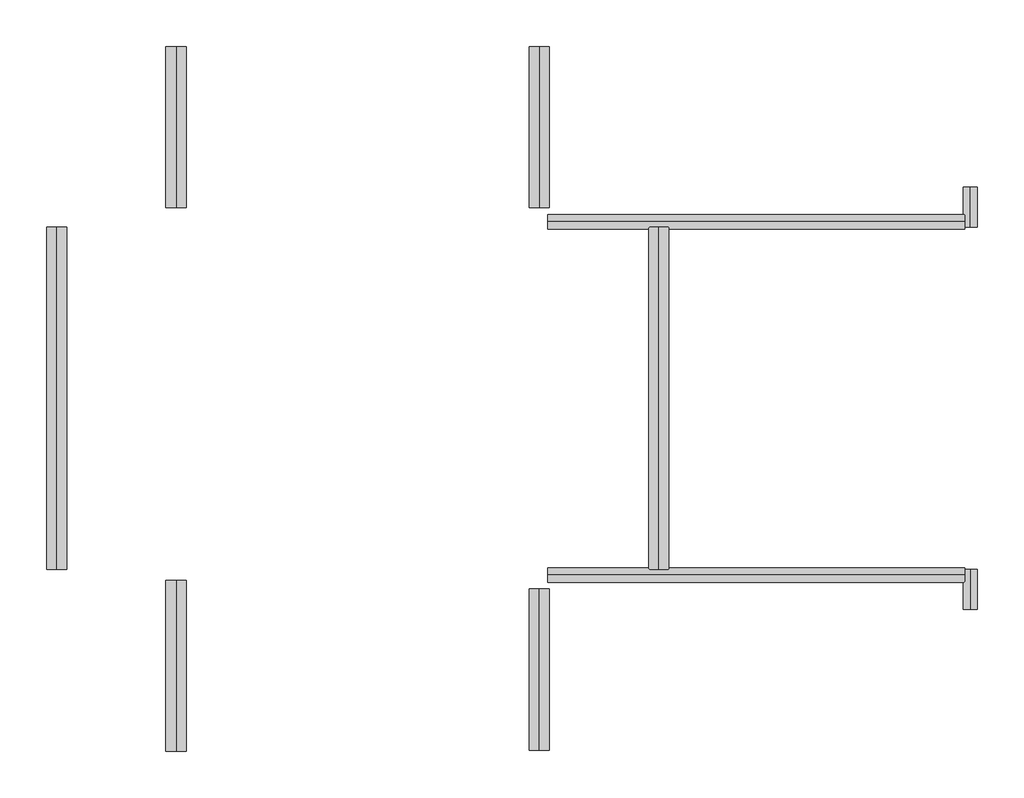
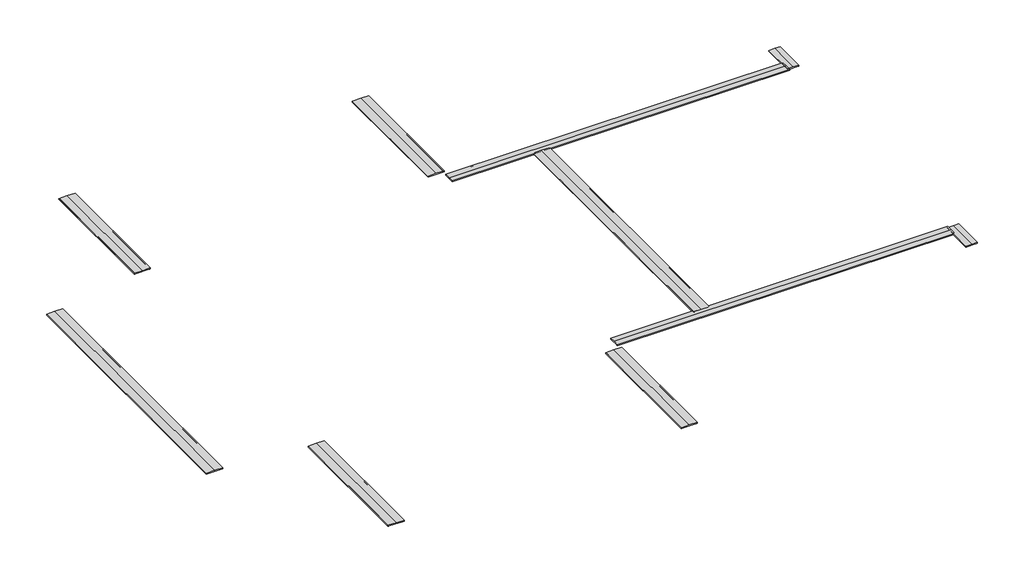
# One storey: 10 proxies.
"""IFC4 building model written with IfcOpenShell, lengths in millimetres."""

from ifc_helpers import new_model, si_unit, frame, origin, place, context, project, spatial, polyline, circle_curve, element, save
from ifc_brep_helpers import plane_surface, revolved_surface, advanced_brep

model = new_model("IFC4")

# Units and contexts
model_context = context("Model", 3, world=origin())
ifc_project = project(units=[si_unit("LENGTHUNIT", "METRE", prefix="MILLI")], contexts=[model_context])

# Site, building, storey
site = spatial("IfcSite", under=ifc_project)
building = spatial("IfcBuilding", under=site)
storey = spatial("IfcBuildingStorey", under=building, Name="AUXILIAR-Peto", Elevation=3030.0)

# Proxies
placement = place(None, origin())
element("IfcBuildingElementProxy", 1, Name="Wall Sweeps", at=placement, inside=storey, context=model_context, shape_type="AdvancedBrep", body=[
    advanced_brep(
    [(-12225.0, -232.5, 3060.0), (-11975.0, -232.5, 3064.3637662), (-11725.0, -232.5, 3060.0), (-11725.0, -232.5, 3030.0), (-11739.8467624, -232.5, 3030.0), (-11754.8467624, -232.5, 3030.0), (-11770.0, -232.5, 3030.0), (-12180.0, -232.5, 3030.0), (-12195.1532376, -232.5, 3030.0), (-12210.1532376, -232.5, 3030.0), (-12225.0, -232.5, 3030.0), (-12225.0, -4252.5, 3060.0), (-12225.0, -4252.5, 3030.0), (-12210.1532376, -4252.5, 3030.0), (-12195.1532376, -4252.5, 3030.0), (-12180.0, -4252.5, 3030.0), (-11770.0, -4252.5, 3030.0), (-11754.8467624, -4252.5, 3030.0), (-11739.8467624, -4252.5, 3030.0), (-11725.0, -4252.5, 3030.0), (-11725.0, -4252.5, 3060.0), (-11975.0, -4252.5, 3064.3637662)],
    [
        (0, 1),
        (1, 2),
        (2, 3),
        (3, 4),
        (4, 5, circle_curve(frame((-11747.3467624, -232.5, 3030.0), z_axis=(0.0, -1.0, 0.0), x_axis=(1.0, 0.0, 0.0)), 7.5)),
        (5, 6),
        (6, 7),
        (7, 8),
        (8, 9, circle_curve(frame((-12202.6532376, -232.5, 3030.0), z_axis=(0.0, -1.0, 0.0), x_axis=(1.0, 0.0, 0.0)), 7.5)),
        (9, 10),
        (10, 0),
        (11, 12),
        (12, 13),
        (13, 14, circle_curve(frame((-12202.6532376, -4252.5, 3030.0), z_axis=(0.0, 1.0, 0.0), x_axis=(1.0, 0.0, 0.0)), 7.5)),
        (14, 15),
        (15, 16),
        (16, 17),
        (17, 18, circle_curve(frame((-11747.3467624, -4252.5, 3030.0), z_axis=(0.0, 1.0, 0.0), x_axis=(1.0, 0.0, 0.0)), 7.5)),
        (18, 19),
        (19, 20),
        (20, 21),
        (21, 11),
        (0, 11),
        (21, 1),
        (20, 2),
        (19, 3),
        (18, 4),
        (17, 5),
        (14, 8),
        (13, 9),
        (12, 10),
    ],
    [
        plane_surface(frame((-12225.9879384, -232.5, 3030.0), z_axis=(0.0, 1.0, 0.0), x_axis=(0.0, 0.0, -1.0))),
        plane_surface(frame((-12225.9879384, -4252.5, 3030.0), z_axis=(0.0, -1.0, 0.0), x_axis=(0.0, 0.0, -1.0))),
        plane_surface(frame((-12225.0, -232.5, 3060.0), z_axis=(-0.01745240643728998, 0.0, 0.9998476951563912), x_axis=(0.0, -1.0, 0.0))),
        plane_surface(frame((-11975.0, -232.5, 3064.3637662), z_axis=(0.017452406437287852, 0.0, 0.9998476951563912), x_axis=(0.0, -1.0, 0.0))),
        plane_surface(frame((-11725.0, -232.5, 3060.0), z_axis=(1.0, 0.0, 0.0), x_axis=(0.0, -1.0, 0.0))),
        plane_surface(frame((-11725.0, -232.5, 3030.0), z_axis=(0.0, 0.0, -1.0), x_axis=(0.0, -1.0, 0.0))),
        revolved_surface(polyline([(-11739.8467624, -4252.5, 3030.0), (-11739.8467624, -232.5, 3030.0)]), (-11747.3467624, -232.5, 3030.0), (0.0, -1.0, 0.0)),
        plane_surface(frame((-11754.8467624, -232.5, 3030.0), z_axis=(0.0, 0.0, -1.0), x_axis=(0.0, -1.0, 0.0))),
        revolved_surface(polyline([(-12195.1532376, -4252.5, 3030.0), (-12195.1532376, -232.5, 3030.0)]), (-12202.6532376, -232.5, 3030.0), (0.0, -1.0, 0.0)),
        plane_surface(frame((-12210.1532376, -232.5, 3030.0), z_axis=(0.0, 0.0, -1.0), x_axis=(0.0, -1.0, 0.0))),
        plane_surface(frame((-12225.0, -232.5, 3030.0), z_axis=(-1.0, 0.0, 0.0), x_axis=(0.0, -1.0, 0.0))),
    ],
    [
        (0, [[1, 2, 3, 4, 5, 6, 7, 8, 9, 10, 11]]),
        (1, [[12, 13, 14, 15, 16, 17, 18, 19, 20, 21, 22]]),
        (2, [[-1, 23, -22, 24]]),
        (3, [[-2, -24, -21, 25]]),
        (4, [[-3, -25, -20, 26]]),
        (5, [[-4, -26, -19, 27]]),
        (6, [[-5, -27, -18, 28]]),
        (7, [[-8, -7, -6, -28, -17, -16, -15, 29]]),
        (8, [[-9, -29, -14, 30]]),
        (9, [[-10, -30, -13, 31]]),
        (10, [[-11, -31, -12, -23]]),
    ],
),
])
element("IfcBuildingElementProxy", 2, Name="Wall Sweeps", at=placement, inside=storey, context=model_context, shape_type="AdvancedBrep", body=[
    advanced_brep(
    [(-20775.0, -232.5, 3060.0), (-20775.0, -232.5, 3030.0), (-20789.8467624, -232.5, 3030.0), (-20804.8467624, -232.5, 3030.0), (-20820.0, -232.5, 3030.0), (-21230.0, -232.5, 3030.0), (-21245.1532376, -232.5, 3030.0), (-21260.1532376, -232.5, 3030.0), (-21275.0, -232.5, 3030.0), (-21275.0, -232.5, 3060.0), (-21025.0, -232.5, 3064.3637662), (-20775.0, -4252.5, 3060.0), (-21025.0, -4252.5, 3064.3637662), (-21275.0, -4252.5, 3060.0), (-21275.0, -4252.5, 3030.0), (-21260.1532376, -4252.5, 3030.0), (-21245.1532376, -4252.5, 3030.0), (-21230.0, -4252.5, 3030.0), (-20820.0, -4252.5, 3030.0), (-20804.8467624, -4252.5, 3030.0), (-20789.8467624, -4252.5, 3030.0), (-20775.0, -4252.5, 3030.0)],
    [
        (0, 1),
        (1, 2),
        (2, 3, circle_curve(frame((-20797.3467624, -232.5, 3030.0), z_axis=(0.0, -1.0, 0.0), x_axis=(-1.0, 0.0, 0.0)), 7.5)),
        (3, 4),
        (4, 5),
        (5, 6),
        (6, 7, circle_curve(frame((-21252.6532376, -232.5, 3030.0), z_axis=(0.0, -1.0, 0.0), x_axis=(-1.0, 0.0, 0.0)), 7.5)),
        (7, 8),
        (8, 9),
        (9, 10),
        (10, 0),
        (11, 12),
        (12, 13),
        (13, 14),
        (14, 15),
        (15, 16, circle_curve(frame((-21252.6532376, -4252.5, 3030.0), z_axis=(0.0, 1.0, 0.0), x_axis=(-1.0, 0.0, 0.0)), 7.5)),
        (16, 17),
        (17, 18),
        (18, 19),
        (19, 20, circle_curve(frame((-20797.3467624, -4252.5, 3030.0), z_axis=(0.0, 1.0, 0.0), x_axis=(-1.0, 0.0, 0.0)), 7.5)),
        (20, 21),
        (21, 11),
        (0, 11),
        (21, 1),
        (20, 2),
        (19, 3),
        (16, 6),
        (15, 7),
        (14, 8),
        (13, 9),
        (12, 10),
    ],
    [
        plane_surface(frame((-21685.9879384, -232.5, 3030.0), z_axis=(0.0, 1.0, 0.0), x_axis=(0.0, 0.0, -1.0))),
        plane_surface(frame((-21685.9879384, -4252.5, 3030.0), z_axis=(0.0, -1.0, 0.0), x_axis=(0.0, 0.0, -1.0))),
        plane_surface(frame((-20775.0, -232.5, 3060.0), z_axis=(1.0, 0.0, 0.0), x_axis=(0.0, -1.0, 0.0))),
        plane_surface(frame((-20775.0, -232.5, 3030.0), z_axis=(0.0, 0.0, -1.0), x_axis=(0.0, -1.0, 0.0))),
        revolved_surface(polyline([(-20804.8467624, -4252.5, 3030.0), (-20804.8467624, -232.5, 3030.0)]), (-20797.3467624, -232.5, 3030.0), (0.0, -1.0, 0.0)),
        plane_surface(frame((-20804.8467624, -232.5, 3030.0), z_axis=(0.0, 0.0, -1.0), x_axis=(0.0, -1.0, 0.0))),
        revolved_surface(polyline([(-21260.1532376, -4252.5, 3030.0), (-21260.1532376, -232.5, 3030.0)]), (-21252.6532376, -232.5, 3030.0), (0.0, -1.0, 0.0)),
        plane_surface(frame((-21260.1532376, -232.5, 3030.0), z_axis=(0.0, 0.0, -1.0), x_axis=(0.0, -1.0, 0.0))),
        plane_surface(frame((-21275.0, -232.5, 3030.0), z_axis=(-1.0, 0.0, 0.0), x_axis=(0.0, -1.0, 0.0))),
        plane_surface(frame((-21275.0, -232.5, 3060.0), z_axis=(-0.017452406437287852, 0.0, 0.9998476951563912), x_axis=(0.0, -1.0, 0.0))),
        plane_surface(frame((-21025.0, -232.5, 3064.3637662), z_axis=(0.01745240643728998, 0.0, 0.9998476951563912), x_axis=(0.0, -1.0, 0.0))),
    ],
    [
        (0, [[1, 2, 3, 4, 5, 6, 7, 8, 9, 10, 11]]),
        (1, [[12, 13, 14, 15, 16, 17, 18, 19, 20, 21, 22]]),
        (2, [[-1, 23, -22, 24]]),
        (3, [[-2, -24, -21, 25]]),
        (4, [[-3, -25, -20, 26]]),
        (5, [[-6, -5, -4, -26, -19, -18, -17, 27]]),
        (6, [[-7, -27, -16, 28]]),
        (7, [[-8, -28, -15, 29]]),
        (8, [[-9, -29, -14, 30]]),
        (9, [[-10, -30, -13, 31]]),
        (10, [[-11, -31, -12, -23]]),
    ],
),
])
element("IfcBuildingElementProxy", 3, Name="Wall Sweeps", at=placement, inside=storey, context=model_context, shape_type="AdvancedBrep", body=[
    advanced_brep(
    [(-12225.0, -17767.5, 3060.0), (-12225.0, -17767.5, 3030.0), (-12210.1532376, -17767.5, 3030.0), (-12195.1532376, -17767.5, 3030.0), (-12180.0, -17767.5, 3030.0), (-11770.0, -17767.5, 3030.0), (-11754.8467624, -17767.5, 3030.0), (-11739.8467624, -17767.5, 3030.0), (-11725.0, -17767.5, 3030.0), (-11725.0, -17767.5, 3060.0), (-11975.0, -17767.5, 3064.3637662), (-12225.0, -13747.5, 3060.0), (-11975.0, -13747.5, 3064.3637662), (-11725.0, -13747.5, 3060.0), (-11725.0, -13747.5, 3030.0), (-11739.8467624, -13747.5, 3030.0), (-11754.8467624, -13747.5, 3030.0), (-11770.0, -13747.5, 3030.0), (-12180.0, -13747.5, 3030.0), (-12195.1532376, -13747.5, 3030.0), (-12210.1532376, -13747.5, 3030.0), (-12225.0, -13747.5, 3030.0)],
    [
        (0, 1),
        (1, 2),
        (2, 3, circle_curve(frame((-12202.6532376, -17767.5, 3030.0), z_axis=(0.0, 1.0, 0.0), x_axis=(1.0, 0.0, 0.0)), 7.5)),
        (3, 4),
        (4, 5),
        (5, 6),
        (6, 7, circle_curve(frame((-11747.3467624, -17767.5, 3030.0), z_axis=(0.0, 1.0, 0.0), x_axis=(1.0, 0.0, 0.0)), 7.5)),
        (7, 8),
        (8, 9),
        (9, 10),
        (10, 0),
        (11, 12),
        (12, 13),
        (13, 14),
        (14, 15),
        (15, 16, circle_curve(frame((-11747.3467624, -13747.5, 3030.0), z_axis=(0.0, -1.0, 0.0), x_axis=(1.0, 0.0, 0.0)), 7.5)),
        (16, 17),
        (17, 18),
        (18, 19),
        (19, 20, circle_curve(frame((-12202.6532376, -13747.5, 3030.0), z_axis=(0.0, -1.0, 0.0), x_axis=(1.0, 0.0, 0.0)), 7.5)),
        (20, 21),
        (21, 11),
        (0, 11),
        (21, 1),
        (20, 2),
        (19, 3),
        (16, 6),
        (15, 7),
        (14, 8),
        (13, 9),
        (12, 10),
    ],
    [
        plane_surface(frame((-12225.9879384, -17767.5, 3030.0), z_axis=(0.0, -1.0, 0.0), x_axis=(0.0, 0.0, 1.0))),
        plane_surface(frame((-12225.9879384, -13747.5, 3030.0), z_axis=(0.0, 1.0, 0.0), x_axis=(0.0, 0.0, 1.0))),
        plane_surface(frame((-12225.0, -17767.5, 3060.0), z_axis=(-1.0, 0.0, 0.0), x_axis=(0.0, 1.0, 0.0))),
        plane_surface(frame((-12225.0, -17767.5, 3030.0), z_axis=(0.0, 0.0, -1.0), x_axis=(0.0, 1.0, 0.0))),
        revolved_surface(polyline([(-12195.1532376, -13747.5, 3030.0), (-12195.1532376, -17767.5, 3030.0)]), (-12202.6532376, -17767.5, 3030.0), (0.0, 1.0, 0.0)),
        plane_surface(frame((-12195.1532376, -17767.5, 3030.0), z_axis=(0.0, 0.0, -1.0), x_axis=(0.0, 1.0, 0.0))),
        revolved_surface(polyline([(-11739.8467624, -13747.5, 3030.0), (-11739.8467624, -17767.5, 3030.0)]), (-11747.3467624, -17767.5, 3030.0), (0.0, 1.0, 0.0)),
        plane_surface(frame((-11739.8467624, -17767.5, 3030.0), z_axis=(0.0, 0.0, -1.0), x_axis=(0.0, 1.0, 0.0))),
        plane_surface(frame((-11725.0, -17767.5, 3030.0), z_axis=(1.0, 0.0, 0.0), x_axis=(0.0, 1.0, 0.0))),
        plane_surface(frame((-11725.0, -17767.5, 3060.0), z_axis=(0.017452406437287852, 0.0, 0.9998476951563912), x_axis=(0.0, 1.0, 0.0))),
        plane_surface(frame((-11975.0, -17767.5, 3064.3637662), z_axis=(-0.01745240643728998, 0.0, 0.9998476951563912), x_axis=(0.0, 1.0, 0.0))),
    ],
    [
        (0, [[1, 2, 3, 4, 5, 6, 7, 8, 9, 10, 11]]),
        (1, [[12, 13, 14, 15, 16, 17, 18, 19, 20, 21, 22]]),
        (2, [[-1, 23, -22, 24]]),
        (3, [[-2, -24, -21, 25]]),
        (4, [[-3, -25, -20, 26]]),
        (5, [[-6, -5, -4, -26, -19, -18, -17, 27]]),
        (6, [[-7, -27, -16, 28]]),
        (7, [[-8, -28, -15, 29]]),
        (8, [[-9, -29, -14, 30]]),
        (9, [[-10, -30, -13, 31]]),
        (10, [[-11, -31, -12, -23]]),
    ],
),
])
element("IfcBuildingElementProxy", 4, Name="Wall Sweeps", at=placement, inside=storey, context=model_context, shape_type="AdvancedBrep", body=[
    advanced_brep(
    [(-23750.0, -13267.5, 3060.0), (-24000.0, -13267.5, 3064.3637662), (-24250.0, -13267.5, 3060.0), (-24250.0, -13267.5, 3030.0), (-24235.1532376, -13267.5, 3030.0), (-24220.1532376, -13267.5, 3030.0), (-24205.0, -13267.5, 3030.0), (-23795.0, -13267.5, 3030.0), (-23779.8467624, -13267.5, 3030.0), (-23764.8467624, -13267.5, 3030.0), (-23750.0, -13267.5, 3030.0), (-23750.0, -4732.5, 3060.0), (-23750.0, -4732.5, 3030.0), (-23764.8467624, -4732.5, 3030.0), (-23779.8467624, -4732.5, 3030.0), (-23795.0, -4732.5, 3030.0), (-24205.0, -4732.5, 3030.0), (-24220.1532376, -4732.5, 3030.0), (-24235.1532376, -4732.5, 3030.0), (-24250.0, -4732.5, 3030.0), (-24250.0, -4732.5, 3060.0), (-24000.0, -4732.5, 3064.3637662)],
    [
        (0, 1),
        (1, 2),
        (2, 3),
        (3, 4),
        (4, 5, circle_curve(frame((-24227.6532376, -13267.5, 3030.0), z_axis=(0.0, 1.0, 0.0), x_axis=(-1.0, 0.0, 0.0)), 7.5)),
        (5, 6),
        (6, 7),
        (7, 8),
        (8, 9, circle_curve(frame((-23772.3467624, -13267.5, 3030.0), z_axis=(0.0, 1.0, 0.0), x_axis=(-1.0, 0.0, 0.0)), 7.5)),
        (9, 10),
        (10, 0),
        (11, 12),
        (12, 13),
        (13, 14, circle_curve(frame((-23772.3467624, -4732.5, 3030.0), z_axis=(0.0, -1.0, 0.0), x_axis=(-1.0, 0.0, 0.0)), 7.5)),
        (14, 15),
        (15, 16),
        (16, 17),
        (17, 18, circle_curve(frame((-24227.6532376, -4732.5, 3030.0), z_axis=(0.0, -1.0, 0.0), x_axis=(-1.0, 0.0, 0.0)), 7.5)),
        (18, 19),
        (19, 20),
        (20, 21),
        (21, 11),
        (0, 11),
        (21, 1),
        (20, 2),
        (19, 3),
        (18, 4),
        (17, 5),
        (14, 8),
        (13, 9),
        (12, 10),
    ],
    [
        plane_surface(frame((-24660.9879384, -13267.5, 3030.0), z_axis=(0.0, -1.0, 0.0), x_axis=(0.0, 0.0, 1.0))),
        plane_surface(frame((-24660.9879384, -4732.5, 3030.0), z_axis=(0.0, 1.0, 0.0), x_axis=(0.0, 0.0, 1.0))),
        plane_surface(frame((-23750.0, -13267.5, 3060.0), z_axis=(0.01745240643728998, 0.0, 0.9998476951563912), x_axis=(0.0, 1.0, 0.0))),
        plane_surface(frame((-24000.0, -13267.5, 3064.3637662), z_axis=(-0.017452406437287852, 0.0, 0.9998476951563912), x_axis=(0.0, 1.0, 0.0))),
        plane_surface(frame((-24250.0, -13267.5, 3060.0), z_axis=(-1.0, 0.0, 0.0), x_axis=(0.0, 1.0, 0.0))),
        plane_surface(frame((-24250.0, -13267.5, 3030.0), z_axis=(0.0, 0.0, -1.0), x_axis=(0.0, 1.0, 0.0))),
        revolved_surface(polyline([(-24235.1532376, -4732.5, 3030.0), (-24235.1532376, -13267.5, 3030.0)]), (-24227.6532376, -13267.5, 3030.0), (0.0, 1.0, 0.0)),
        plane_surface(frame((-24220.1532376, -13267.5, 3030.0), z_axis=(0.0, 0.0, -1.0), x_axis=(0.0, 1.0, 0.0))),
        revolved_surface(polyline([(-23779.8467624, -4732.5, 3030.0), (-23779.8467624, -13267.5, 3030.0)]), (-23772.3467624, -13267.5, 3030.0), (0.0, 1.0, 0.0)),
        plane_surface(frame((-23764.8467624, -13267.5, 3030.0), z_axis=(0.0, 0.0, -1.0), x_axis=(0.0, 1.0, 0.0))),
        plane_surface(frame((-23750.0, -13267.5, 3030.0), z_axis=(1.0, 0.0, 0.0), x_axis=(0.0, 1.0, 0.0))),
    ],
    [
        (0, [[1, 2, 3, 4, 5, 6, 7, 8, 9, 10, 11]]),
        (1, [[12, 13, 14, 15, 16, 17, 18, 19, 20, 21, 22]]),
        (2, [[-1, 23, -22, 24]]),
        (3, [[-2, -24, -21, 25]]),
        (4, [[-3, -25, -20, 26]]),
        (5, [[-4, -26, -19, 27]]),
        (6, [[-5, -27, -18, 28]]),
        (7, [[-8, -7, -6, -28, -17, -16, -15, 29]]),
        (8, [[-9, -29, -14, 30]]),
        (9, [[-10, -30, -13, 31]]),
        (10, [[-11, -31, -12, -23]]),
    ],
),
])
element("IfcBuildingElementProxy", 5, Name="Wall Sweeps", at=placement, inside=storey, context=model_context, shape_type="AdvancedBrep", body=[
    advanced_brep(
    [(-9250.0, -13267.5, 3060.0), (-9250.0, -13267.5, 3030.0), (-9235.1532376, -13267.5, 3030.0), (-9220.1532376, -13267.5, 3030.0), (-9205.0, -13267.5, 3030.0), (-8795.0, -13267.5, 3030.0), (-8779.8467624, -13267.5, 3030.0), (-8764.8467624, -13267.5, 3030.0), (-8750.0, -13267.5, 3030.0), (-8750.0, -13267.5, 3060.0), (-9000.0, -13267.5, 3064.3637662), (-9250.0, -4732.5, 3060.0), (-9000.0, -4732.5, 3064.3637662), (-8750.0, -4732.5, 3060.0), (-8750.0, -4732.5, 3030.0), (-8764.8467624, -4732.5, 3030.0), (-8779.8467624, -4732.5, 3030.0), (-8795.0, -4732.5, 3030.0), (-9205.0, -4732.5, 3030.0), (-9220.1532376, -4732.5, 3030.0), (-9235.1532376, -4732.5, 3030.0), (-9250.0, -4732.5, 3030.0)],
    [
        (0, 1),
        (1, 2),
        (2, 3, circle_curve(frame((-9227.6532376, -13267.5, 3030.0), z_axis=(0.0, 1.0, 0.0), x_axis=(1.0, 0.0, 0.0)), 7.5)),
        (3, 4),
        (4, 5),
        (5, 6),
        (6, 7, circle_curve(frame((-8772.3467624, -13267.5, 3030.0), z_axis=(0.0, 1.0, 0.0), x_axis=(1.0, 0.0, 0.0)), 7.5)),
        (7, 8),
        (8, 9),
        (9, 10),
        (10, 0),
        (11, 12),
        (12, 13),
        (13, 14),
        (14, 15),
        (15, 16, circle_curve(frame((-8772.3467624, -4732.5, 3030.0), z_axis=(0.0, -1.0, 0.0), x_axis=(1.0, 0.0, 0.0)), 7.5)),
        (16, 17),
        (17, 18),
        (18, 19),
        (19, 20, circle_curve(frame((-9227.6532376, -4732.5, 3030.0), z_axis=(0.0, -1.0, 0.0), x_axis=(1.0, 0.0, 0.0)), 7.5)),
        (20, 21),
        (21, 11),
        (0, 11),
        (21, 1),
        (20, 2),
        (19, 3),
        (16, 6),
        (15, 7),
        (14, 8),
        (13, 9),
        (12, 10),
    ],
    [
        plane_surface(frame((-9250.9879384, -13267.5, 3030.0), z_axis=(0.0, -1.0, 0.0), x_axis=(0.0, 0.0, 1.0))),
        plane_surface(frame((-9250.9879384, -4732.5, 3030.0), z_axis=(0.0, 1.0, 0.0), x_axis=(0.0, 0.0, 1.0))),
        plane_surface(frame((-9250.0, -13267.5, 3060.0), z_axis=(-1.0, 0.0, 0.0), x_axis=(0.0, 1.0, 0.0))),
        plane_surface(frame((-9250.0, -13267.5, 3030.0), z_axis=(0.0, 0.0, -1.0), x_axis=(0.0, 1.0, 0.0))),
        revolved_surface(polyline([(-9220.1532376, -4732.5, 3030.0), (-9220.1532376, -13267.5, 3030.0)]), (-9227.6532376, -13267.5, 3030.0), (0.0, 1.0, 0.0)),
        plane_surface(frame((-9220.1532376, -13267.5, 3030.0), z_axis=(0.0, 0.0, -1.0), x_axis=(0.0, 1.0, 0.0))),
        revolved_surface(polyline([(-8764.8467624, -4732.5, 3030.0), (-8764.8467624, -13267.5, 3030.0)]), (-8772.3467624, -13267.5, 3030.0), (0.0, 1.0, 0.0)),
        plane_surface(frame((-8764.8467624, -13267.5, 3030.0), z_axis=(0.0, 0.0, -1.0), x_axis=(0.0, 1.0, 0.0))),
        plane_surface(frame((-8750.0, -13267.5, 3030.0), z_axis=(1.0, 0.0, 0.0), x_axis=(0.0, 1.0, 0.0))),
        plane_surface(frame((-8750.0, -13267.5, 3060.0), z_axis=(0.017452406437287852, 0.0, 0.9998476951563912), x_axis=(0.0, 1.0, 0.0))),
        plane_surface(frame((-9000.0, -13267.5, 3064.3637662), z_axis=(-0.01745240643728998, 0.0, 0.9998476951563912), x_axis=(0.0, 1.0, 0.0))),
    ],
    [
        (0, [[1, 2, 3, 4, 5, 6, 7, 8, 9, 10, 11]]),
        (1, [[12, 13, 14, 15, 16, 17, 18, 19, 20, 21, 22]]),
        (2, [[-1, 23, -22, 24]]),
        (3, [[-2, -24, -21, 25]]),
        (4, [[-3, -25, -20, 26]]),
        (5, [[-6, -5, -4, -26, -19, -18, -17, 27]]),
        (6, [[-7, -27, -16, 28]]),
        (7, [[-8, -28, -15, 29]]),
        (8, [[-9, -29, -14, 30]]),
        (9, [[-10, -30, -13, 31]]),
        (10, [[-11, -31, -12, -23]]),
    ],
),
])
element("IfcBuildingElementProxy", 6, Name="Wall Sweeps", at=placement, inside=storey, context=model_context, shape_type="AdvancedBrep", body=[
    advanced_brep(
    [(-11770.0, -13222.5, 3060.0), (-11770.0, -13222.5, 3030.0), (-11770.0, -13237.3467624, 3030.0), (-11770.0, -13252.3467624, 3030.0), (-11770.0, -13267.5, 3030.0), (-11770.0, -13537.5, 3030.0), (-11770.0, -13552.6532376, 3030.0), (-11770.0, -13567.6532376, 3030.0), (-11770.0, -13582.5, 3030.0), (-11770.0, -13582.5, 3060.0), (-11770.0, -13402.5, 3063.1419117), (-1380.0, -13222.5, 3060.0), (-1380.0, -13402.5, 3063.1419117), (-1380.0, -13582.5, 3060.0), (-1380.0, -13582.5, 3030.0), (-1380.0, -13567.6532376, 3030.0), (-1380.0, -13552.6532376, 3030.0), (-1380.0, -13252.3467624, 3030.0), (-1380.0, -13237.3467624, 3030.0), (-1380.0, -13222.5, 3030.0)],
    [
        (0, 1),
        (1, 2),
        (2, 3, circle_curve(frame((-11770.0, -13244.8467624, 3030.0), z_axis=(1.0, 0.0, 0.0), x_axis=(0.0, -1.0, 0.0)), 7.5)),
        (3, 4),
        (4, 5),
        (5, 6),
        (6, 7, circle_curve(frame((-11770.0, -13560.1532376, 3030.0), z_axis=(1.0, 0.0, 0.0), x_axis=(0.0, -1.0, 0.0)), 7.5)),
        (7, 8),
        (8, 9),
        (9, 10),
        (10, 0),
        (11, 12),
        (12, 13),
        (13, 14),
        (14, 15),
        (15, 16, circle_curve(frame((-1380.0, -13560.1532376, 3030.0), z_axis=(-1.0, 0.0, 0.0), x_axis=(0.0, -1.0, 0.0)), 7.5)),
        (16, 17),
        (17, 18, circle_curve(frame((-1380.0, -13244.8467624, 3030.0), z_axis=(-1.0, 0.0, 0.0), x_axis=(0.0, -1.0, 0.0)), 7.5)),
        (18, 19),
        (19, 11),
        (0, 11),
        (19, 1),
        (18, 2),
        (17, 3),
        (16, 6),
        (15, 7),
        (14, 8),
        (13, 9),
        (12, 10),
    ],
    [
        plane_surface(frame((-11770.0, -13537.5, 2713.5746534), z_axis=(-1.0, 0.0, 0.0), x_axis=(0.0, 1.0, 0.0))),
        plane_surface(frame((-1380.0, -13537.5, 2713.5746534), z_axis=(1.0, 0.0, 0.0), x_axis=(0.0, 1.0, 0.0))),
        plane_surface(frame((-11770.0, -13222.5, 3060.0), z_axis=(0.0, 1.0, 0.0), x_axis=(1.0, 0.0, 0.0))),
        plane_surface(frame((-11770.0, -13222.5, 3030.0), z_axis=(0.0, 0.0, -1.0), x_axis=(1.0, 0.0, 0.0))),
        revolved_surface(polyline([(-1380.0, -13252.3467624, 3030.0), (-11770.0, -13252.3467624, 3030.0)]), (-11770.0, -13244.8467624, 3030.0), (1.0, 0.0, 0.0)),
        plane_surface(frame((-11770.0, -13252.3467624, 3030.0), z_axis=(0.0, 0.0, -1.0), x_axis=(1.0, 0.0, 0.0))),
        revolved_surface(polyline([(-1380.0, -13567.6532376, 3030.0), (-11770.0, -13567.6532376, 3030.0)]), (-11770.0, -13560.1532376, 3030.0), (1.0, 0.0, 0.0)),
        plane_surface(frame((-11770.0, -13567.6532376, 3030.0), z_axis=(0.0, 0.0, -1.0), x_axis=(1.0, 0.0, 0.0))),
        plane_surface(frame((-11770.0, -13582.5, 3030.0), z_axis=(0.0, -1.0, 0.0), x_axis=(1.0, 0.0, 0.0))),
        plane_surface(frame((-11770.0, -13582.5, 3060.0), z_axis=(0.0, -0.01745240643728671, 0.9998476951563913), x_axis=(1.0, 0.0, 0.0))),
        plane_surface(frame((-11770.0, -13402.5, 3063.1419117), z_axis=(0.0, 0.01745240643728026, 0.9998476951563914), x_axis=(1.0, 0.0, 0.0))),
    ],
    [
        (0, [[1, 2, 3, 4, 5, 6, 7, 8, 9, 10, 11]]),
        (1, [[12, 13, 14, 15, 16, 17, 18, 19, 20]]),
        (2, [[-1, 21, -20, 22]]),
        (3, [[-2, -22, -19, 23]]),
        (4, [[-3, -23, -18, 24]]),
        (5, [[-6, -5, -4, -24, -17, 25]]),
        (6, [[-7, -25, -16, 26]]),
        (7, [[-8, -26, -15, 27]]),
        (8, [[-9, -27, -14, 28]]),
        (9, [[-10, -28, -13, 29]]),
        (10, [[-11, -29, -12, -21]]),
    ],
),
])
element("IfcBuildingElementProxy", 7, Name="Wall Sweeps", at=placement, inside=storey, context=model_context, shape_type="AdvancedBrep", body=[
    advanced_brep(
    [(-1425.0, -13267.5, 3060.0), (-1245.0, -13267.5, 3063.1419117), (-1065.0, -13267.5, 3060.0), (-1065.0, -13267.5, 3030.0), (-1079.8467624, -13267.5, 3030.0), (-1094.8467624, -13267.5, 3030.0), (-1395.1532376, -13267.5, 3030.0), (-1410.1532376, -13267.5, 3030.0), (-1425.0, -13267.5, 3030.0), (-1425.0, -14257.5, 3060.0), (-1425.0, -14257.5, 3030.0), (-1410.1532376, -14257.5, 3030.0), (-1395.1532376, -14257.5, 3030.0), (-1380.0, -14257.5, 3030.0), (-1110.0, -14257.5, 3030.0), (-1094.8467624, -14257.5, 3030.0), (-1079.8467624, -14257.5, 3030.0), (-1065.0, -14257.5, 3030.0), (-1065.0, -14257.5, 3060.0), (-1245.0, -14257.5, 3063.1419117)],
    [
        (0, 1),
        (1, 2),
        (2, 3),
        (3, 4),
        (4, 5, circle_curve(frame((-1087.3467624, -13267.5, 3030.0), z_axis=(0.0, -1.0, 0.0), x_axis=(1.0, 0.0, 0.0)), 7.5)),
        (5, 6),
        (6, 7, circle_curve(frame((-1402.6532376, -13267.5, 3030.0), z_axis=(0.0, -1.0, 0.0), x_axis=(1.0, 0.0, 0.0)), 7.5)),
        (7, 8),
        (8, 0),
        (9, 10),
        (10, 11),
        (11, 12, circle_curve(frame((-1402.6532376, -14257.5, 3030.0), z_axis=(0.0, 1.0, 0.0), x_axis=(1.0, 0.0, 0.0)), 7.5)),
        (12, 13),
        (13, 14),
        (14, 15),
        (15, 16, circle_curve(frame((-1087.3467624, -14257.5, 3030.0), z_axis=(0.0, 1.0, 0.0), x_axis=(1.0, 0.0, 0.0)), 7.5)),
        (16, 17),
        (17, 18),
        (18, 19),
        (19, 9),
        (0, 9),
        (19, 1),
        (18, 2),
        (17, 3),
        (16, 4),
        (15, 5),
        (12, 6),
        (11, 7),
        (10, 8),
    ],
    [
        plane_surface(frame((-1426.4253466, -13267.5, 3030.0), z_axis=(0.0, 1.0, 0.0), x_axis=(0.0, 0.0, -1.0))),
        plane_surface(frame((-1426.4253466, -14257.5, 3030.0), z_axis=(0.0, -1.0, 0.0), x_axis=(0.0, 0.0, -1.0))),
        plane_surface(frame((-1425.0, -13267.5, 3060.0), z_axis=(-0.01745240643728026, 0.0, 0.9998476951563914), x_axis=(0.0, -1.0, 0.0))),
        plane_surface(frame((-1245.0, -13267.5, 3063.1419117), z_axis=(0.01745240643728671, 0.0, 0.9998476951563913), x_axis=(0.0, -1.0, 0.0))),
        plane_surface(frame((-1065.0, -13267.5, 3060.0), z_axis=(1.0, 0.0, 0.0), x_axis=(0.0, -1.0, 0.0))),
        plane_surface(frame((-1065.0, -13267.5, 3030.0), z_axis=(0.0, 0.0, -1.0), x_axis=(0.0, -1.0, 0.0))),
        revolved_surface(polyline([(-1079.8467624, -14257.5, 3030.0), (-1079.8467624, -13267.5, 3030.0)]), (-1087.3467624, -13267.5, 3030.0), (0.0, -1.0, 0.0)),
        plane_surface(frame((-1094.8467624, -13267.5, 3030.0), z_axis=(0.0, 0.0, -1.0), x_axis=(0.0, -1.0, 0.0))),
        revolved_surface(polyline([(-1395.1532376, -14257.5, 3030.0), (-1395.1532376, -13267.5, 3030.0)]), (-1402.6532376, -13267.5, 3030.0), (0.0, -1.0, 0.0)),
        plane_surface(frame((-1410.1532376, -13267.5, 3030.0), z_axis=(0.0, 0.0, -1.0), x_axis=(0.0, -1.0, 0.0))),
        plane_surface(frame((-1425.0, -13267.5, 3030.0), z_axis=(-1.0, 0.0, 0.0), x_axis=(0.0, -1.0, 0.0))),
    ],
    [
        (0, [[1, 2, 3, 4, 5, 6, 7, 8, 9]]),
        (1, [[10, 11, 12, 13, 14, 15, 16, 17, 18, 19, 20]]),
        (2, [[-1, 21, -20, 22]]),
        (3, [[-2, -22, -19, 23]]),
        (4, [[-3, -23, -18, 24]]),
        (5, [[-4, -24, -17, 25]]),
        (6, [[-5, -25, -16, 26]]),
        (7, [[-6, -26, -15, -14, -13, 27]]),
        (8, [[-7, -27, -12, 28]]),
        (9, [[-8, -28, -11, 29]]),
        (10, [[-9, -29, -10, -21]]),
    ],
),
])
element("IfcBuildingElementProxy", 8, Name="Wall Sweeps", at=placement, inside=storey, context=model_context, shape_type="AdvancedBrep", body=[
    advanced_brep(
    [(-11770.0, -4777.5, 3060.0), (-11770.0, -4597.5, 3063.1419117), (-11770.0, -4417.5, 3060.0), (-11770.0, -4417.5, 3030.0), (-11770.0, -4432.3467624, 3030.0), (-11770.0, -4447.3467624, 3030.0), (-11770.0, -4462.5, 3030.0), (-11770.0, -4732.5, 3030.0), (-11770.0, -4747.6532376, 3030.0), (-11770.0, -4762.6532376, 3030.0), (-11770.0, -4777.5, 3030.0), (-1380.0, -4777.5, 3060.0), (-1380.0, -4777.5, 3030.0), (-1380.0, -4762.6532376, 3030.0), (-1380.0, -4747.6532376, 3030.0), (-1380.0, -4447.3467624, 3030.0), (-1380.0, -4432.3467624, 3030.0), (-1380.0, -4417.5, 3030.0), (-1380.0, -4417.5, 3060.0), (-1380.0, -4597.5, 3063.1419117)],
    [
        (0, 1),
        (1, 2),
        (2, 3),
        (3, 4),
        (4, 5, circle_curve(frame((-11770.0, -4439.8467624, 3030.0), z_axis=(1.0, 0.0, 0.0), x_axis=(0.0, 1.0, 0.0)), 7.5)),
        (5, 6),
        (6, 7),
        (7, 8),
        (8, 9, circle_curve(frame((-11770.0, -4755.1532376, 3030.0), z_axis=(1.0, 0.0, 0.0), x_axis=(0.0, 1.0, 0.0)), 7.5)),
        (9, 10),
        (10, 0),
        (11, 12),
        (12, 13),
        (13, 14, circle_curve(frame((-1380.0, -4755.1532376, 3030.0), z_axis=(-1.0, 0.0, 0.0), x_axis=(0.0, 1.0, 0.0)), 7.5)),
        (14, 15),
        (15, 16, circle_curve(frame((-1380.0, -4439.8467624, 3030.0), z_axis=(-1.0, 0.0, 0.0), x_axis=(0.0, 1.0, 0.0)), 7.5)),
        (16, 17),
        (17, 18),
        (18, 19),
        (19, 11),
        (0, 11),
        (19, 1),
        (18, 2),
        (17, 3),
        (16, 4),
        (15, 5),
        (14, 8),
        (13, 9),
        (12, 10),
    ],
    [
        plane_surface(frame((-11770.0, -4462.5, 2713.5746534), z_axis=(-1.0, 0.0, 0.0), x_axis=(0.0, 1.0, 0.0))),
        plane_surface(frame((-1380.0, -4462.5, 2713.5746534), z_axis=(1.0, 0.0, 0.0), x_axis=(0.0, 1.0, 0.0))),
        plane_surface(frame((-11770.0, -4777.5, 3060.0), z_axis=(0.0, -0.01745240643728026, 0.9998476951563914), x_axis=(1.0, 0.0, 0.0))),
        plane_surface(frame((-11770.0, -4597.5, 3063.1419117), z_axis=(0.0, 0.01745240643728671, 0.9998476951563913), x_axis=(1.0, 0.0, 0.0))),
        plane_surface(frame((-11770.0, -4417.5, 3060.0), z_axis=(0.0, 1.0, 0.0), x_axis=(1.0, 0.0, 0.0))),
        plane_surface(frame((-11770.0, -4417.5, 3030.0), z_axis=(0.0, 0.0, -1.0), x_axis=(1.0, 0.0, 0.0))),
        revolved_surface(polyline([(-1380.0, -4432.3467624, 3030.0), (-11770.0, -4432.3467624, 3030.0)]), (-11770.0, -4439.8467624, 3030.0), (1.0, 0.0, 0.0)),
        plane_surface(frame((-11770.0, -4447.3467624, 3030.0), z_axis=(0.0, 0.0, -1.0), x_axis=(1.0, 0.0, 0.0))),
        revolved_surface(polyline([(-1380.0, -4747.6532376, 3030.0), (-11770.0, -4747.6532376, 3030.0)]), (-11770.0, -4755.1532376, 3030.0), (1.0, 0.0, 0.0)),
        plane_surface(frame((-11770.0, -4762.6532376, 3030.0), z_axis=(0.0, 0.0, -1.0), x_axis=(1.0, 0.0, 0.0))),
        plane_surface(frame((-11770.0, -4777.5, 3030.0), z_axis=(0.0, -1.0, 0.0), x_axis=(1.0, 0.0, 0.0))),
    ],
    [
        (0, [[1, 2, 3, 4, 5, 6, 7, 8, 9, 10, 11]]),
        (1, [[12, 13, 14, 15, 16, 17, 18, 19, 20]]),
        (2, [[-1, 21, -20, 22]]),
        (3, [[-2, -22, -19, 23]]),
        (4, [[-3, -23, -18, 24]]),
        (5, [[-4, -24, -17, 25]]),
        (6, [[-5, -25, -16, 26]]),
        (7, [[-8, -7, -6, -26, -15, 27]]),
        (8, [[-9, -27, -14, 28]]),
        (9, [[-10, -28, -13, 29]]),
        (10, [[-11, -29, -12, -21]]),
    ],
),
])
element("IfcBuildingElementProxy", 9, Name="Wall Sweeps", at=placement, inside=storey, context=model_context, shape_type="AdvancedBrep", body=[
    advanced_brep(
    [(-1425.0, -4732.5, 3060.0), (-1425.0, -4732.5, 3030.0), (-1410.1532376, -4732.5, 3030.0), (-1395.1532376, -4732.5, 3030.0), (-1094.8467624, -4732.5, 3030.0), (-1079.8467624, -4732.5, 3030.0), (-1065.0, -4732.5, 3030.0), (-1065.0, -4732.5, 3060.0), (-1245.0, -4732.5, 3063.1419117), (-1425.0, -3742.5, 3060.0), (-1245.0, -3742.5, 3063.1419117), (-1065.0, -3742.5, 3060.0), (-1065.0, -3742.5, 3030.0), (-1079.8467624, -3742.5, 3030.0), (-1094.8467624, -3742.5, 3030.0), (-1110.0, -3742.5, 3030.0), (-1380.0, -3742.5, 3030.0), (-1395.1532376, -3742.5, 3030.0), (-1410.1532376, -3742.5, 3030.0), (-1425.0, -3742.5, 3030.0)],
    [
        (0, 1),
        (1, 2),
        (2, 3, circle_curve(frame((-1402.6532376, -4732.5, 3030.0), z_axis=(0.0, 1.0, 0.0), x_axis=(1.0, 0.0, 0.0)), 7.5)),
        (3, 4),
        (4, 5, circle_curve(frame((-1087.3467624, -4732.5, 3030.0), z_axis=(0.0, 1.0, 0.0), x_axis=(1.0, 0.0, 0.0)), 7.5)),
        (5, 6),
        (6, 7),
        (7, 8),
        (8, 0),
        (9, 10),
        (10, 11),
        (11, 12),
        (12, 13),
        (13, 14, circle_curve(frame((-1087.3467624, -3742.5, 3030.0), z_axis=(0.0, -1.0, 0.0), x_axis=(1.0, 0.0, 0.0)), 7.5)),
        (14, 15),
        (15, 16),
        (16, 17),
        (17, 18, circle_curve(frame((-1402.6532376, -3742.5, 3030.0), z_axis=(0.0, -1.0, 0.0), x_axis=(1.0, 0.0, 0.0)), 7.5)),
        (18, 19),
        (19, 9),
        (0, 9),
        (19, 1),
        (18, 2),
        (17, 3),
        (14, 4),
        (13, 5),
        (12, 6),
        (11, 7),
        (10, 8),
    ],
    [
        plane_surface(frame((-1426.4253466, -4732.5, 3030.0), z_axis=(0.0, -1.0, 0.0), x_axis=(0.0, 0.0, 1.0))),
        plane_surface(frame((-1426.4253466, -3742.5, 3030.0), z_axis=(0.0, 1.0, 0.0), x_axis=(0.0, 0.0, 1.0))),
        plane_surface(frame((-1425.0, -4732.5, 3060.0), z_axis=(-1.0, 0.0, 0.0), x_axis=(0.0, 1.0, 0.0))),
        plane_surface(frame((-1425.0, -4732.5, 3030.0), z_axis=(0.0, 0.0, -1.0), x_axis=(0.0, 1.0, 0.0))),
        revolved_surface(polyline([(-1395.1532376, -3742.5, 3030.0), (-1395.1532376, -4732.5, 3030.0)]), (-1402.6532376, -4732.5, 3030.0), (0.0, 1.0, 0.0)),
        plane_surface(frame((-1395.1532376, -4732.5, 3030.0), z_axis=(0.0, 0.0, -1.0), x_axis=(0.0, 1.0, 0.0))),
        revolved_surface(polyline([(-1079.8467624, -3742.5, 3030.0), (-1079.8467624, -4732.5, 3030.0)]), (-1087.3467624, -4732.5, 3030.0), (0.0, 1.0, 0.0)),
        plane_surface(frame((-1079.8467624, -4732.5, 3030.0), z_axis=(0.0, 0.0, -1.0), x_axis=(0.0, 1.0, 0.0))),
        plane_surface(frame((-1065.0, -4732.5, 3030.0), z_axis=(1.0, 0.0, 0.0), x_axis=(0.0, 1.0, 0.0))),
        plane_surface(frame((-1065.0, -4732.5, 3060.0), z_axis=(0.01745240643728671, 0.0, 0.9998476951563913), x_axis=(0.0, 1.0, 0.0))),
        plane_surface(frame((-1245.0, -4732.5, 3063.1419117), z_axis=(-0.01745240643728026, 0.0, 0.9998476951563914), x_axis=(0.0, 1.0, 0.0))),
    ],
    [
        (0, [[1, 2, 3, 4, 5, 6, 7, 8, 9]]),
        (1, [[10, 11, 12, 13, 14, 15, 16, 17, 18, 19, 20]]),
        (2, [[-1, 21, -20, 22]]),
        (3, [[-2, -22, -19, 23]]),
        (4, [[-3, -23, -18, 24]]),
        (5, [[-4, -24, -17, -16, -15, 25]]),
        (6, [[-5, -25, -14, 26]]),
        (7, [[-6, -26, -13, 27]]),
        (8, [[-7, -27, -12, 28]]),
        (9, [[-8, -28, -11, 29]]),
        (10, [[-9, -29, -10, -21]]),
    ],
),
])
element("IfcBuildingElementProxy", 10, Name="Wall Sweeps", at=placement, inside=storey, context=model_context, shape_type="AdvancedBrep", body=[
    advanced_brep(
    [(-20775.0, -17797.5, 3060.0), (-21025.0, -17797.5, 3064.3637662), (-21275.0, -17797.5, 3060.0), (-21275.0, -17797.5, 3030.0), (-21260.1532376, -17797.5, 3030.0), (-21245.1532376, -17797.5, 3030.0), (-21230.0, -17797.5, 3030.0), (-20820.0, -17797.5, 3030.0), (-20804.8467624, -17797.5, 3030.0), (-20789.8467624, -17797.5, 3030.0), (-20775.0, -17797.5, 3030.0), (-20775.0, -13537.5, 3060.0), (-20775.0, -13537.5, 3030.0), (-20789.8467624, -13537.5, 3030.0), (-20804.8467624, -13537.5, 3030.0), (-20820.0, -13537.5, 3030.0), (-21230.0, -13537.5, 3030.0), (-21245.1532376, -13537.5, 3030.0), (-21260.1532376, -13537.5, 3030.0), (-21275.0, -13537.5, 3030.0), (-21275.0, -13537.5, 3060.0), (-21025.0, -13537.5, 3064.3637662)],
    [
        (0, 1),
        (1, 2),
        (2, 3),
        (3, 4),
        (4, 5, circle_curve(frame((-21252.6532376, -17797.5, 3030.0), z_axis=(0.0, 1.0, 0.0), x_axis=(-1.0, 0.0, 0.0)), 7.5)),
        (5, 6),
        (6, 7),
        (7, 8),
        (8, 9, circle_curve(frame((-20797.3467624, -17797.5, 3030.0), z_axis=(0.0, 1.0, 0.0), x_axis=(-1.0, 0.0, 0.0)), 7.5)),
        (9, 10),
        (10, 0),
        (11, 12),
        (12, 13),
        (13, 14, circle_curve(frame((-20797.3467624, -13537.5, 3030.0), z_axis=(0.0, -1.0, 0.0), x_axis=(-1.0, 0.0, 0.0)), 7.5)),
        (14, 15),
        (15, 16),
        (16, 17),
        (17, 18, circle_curve(frame((-21252.6532376, -13537.5, 3030.0), z_axis=(0.0, -1.0, 0.0), x_axis=(-1.0, 0.0, 0.0)), 7.5)),
        (18, 19),
        (19, 20),
        (20, 21),
        (21, 11),
        (10, 12),
        (11, 0),
        (9, 13),
        (8, 14),
        (5, 17),
        (4, 18),
        (3, 19),
        (2, 20),
        (1, 21),
    ],
    [
        plane_surface(frame((-21685.9879384, -17797.5, 3030.0), z_axis=(0.0, -1.0, 0.0), x_axis=(0.0, 0.0, 1.0))),
        plane_surface(frame((-21685.9879384, -13537.5, 3030.0), z_axis=(0.0, 1.0, 0.0), x_axis=(0.0, 0.0, 1.0))),
        plane_surface(frame((-20775.0, -17797.5, 3030.0), z_axis=(1.0, 0.0, 0.0), x_axis=(0.0, 1.0, 0.0))),
        plane_surface(frame((-20789.8467624, -17797.5, 3030.0), z_axis=(0.0, 0.0, -1.0), x_axis=(0.0, 1.0, 0.0))),
        revolved_surface(polyline([(-20804.8467624, -13537.5, 3030.0), (-20804.8467624, -17797.5, 3030.0)]), (-20797.3467624, -17797.5, 3030.0), (0.0, 1.0, 0.0)),
        plane_surface(frame((-21245.1532376, -17797.5, 3030.0), z_axis=(0.0, 0.0, -1.0), x_axis=(0.0, 1.0, 0.0))),
        revolved_surface(polyline([(-21260.1532376, -13537.5, 3030.0), (-21260.1532376, -17797.5, 3030.0)]), (-21252.6532376, -17797.5, 3030.0), (0.0, 1.0, 0.0)),
        plane_surface(frame((-21275.0, -17797.5, 3030.0), z_axis=(0.0, 0.0, -1.0), x_axis=(0.0, 1.0, 0.0))),
        plane_surface(frame((-21275.0, -17797.5, 3060.0), z_axis=(-1.0, 0.0, 0.0), x_axis=(0.0, 1.0, 0.0))),
        plane_surface(frame((-21025.0, -17797.5, 3064.3637662), z_axis=(-0.017452406437287852, 0.0, 0.9998476951563912), x_axis=(0.0, 1.0, 0.0))),
        plane_surface(frame((-20775.0, -17797.5, 3060.0), z_axis=(0.01745240643728998, 0.0, 0.9998476951563912), x_axis=(0.0, 1.0, 0.0))),
    ],
    [
        (0, [[1, 2, 3, 4, 5, 6, 7, 8, 9, 10, 11]]),
        (1, [[12, 13, 14, 15, 16, 17, 18, 19, 20, 21, 22]]),
        (2, [[-11, 23, -12, 24]]),
        (3, [[-10, 25, -13, -23]]),
        (4, [[-9, 26, -14, -25]]),
        (5, [[-8, -7, -6, 27, -17, -16, -15, -26]]),
        (6, [[-5, 28, -18, -27]]),
        (7, [[-4, 29, -19, -28]]),
        (8, [[-3, 30, -20, -29]]),
        (9, [[-2, 31, -21, -30]]),
        (10, [[-1, -24, -22, -31]]),
    ],
),
])

save(model, "model.ifc")

# Revit data of these elements
# Elements 1, 2, 3, 4, 5, 6, 7, 8, 9, 10 (IfcBuildingElementProxy)
#   Phase Created = Nueva construcción
#   Materials on its faces: "Muro por defecto"
# Materials
#   "Muro por defecto": class "Varios", colour RGB 212 212 212, transparency 0, Cost = 0
